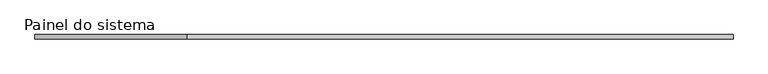
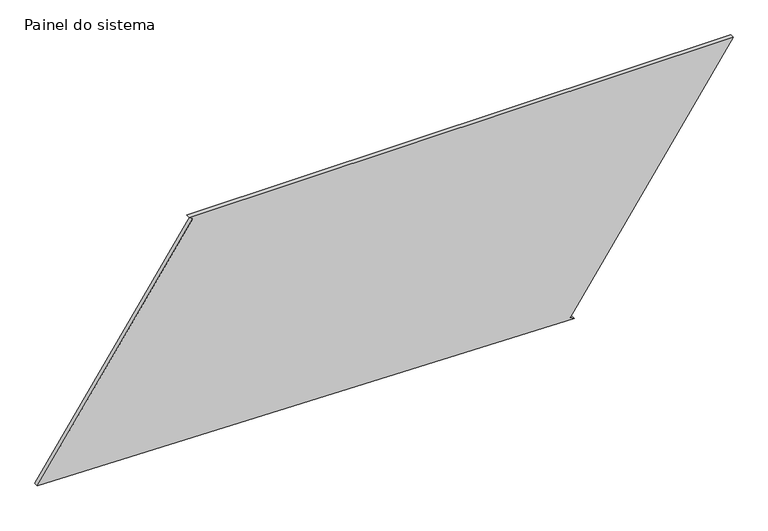
"""IFC4 building model written with IfcOpenShell, lengths in millimetres: plate geometry, Painel do sistema : Envidraçado."""

from ifc_helpers import new_model, si_unit, frame, origin, place, context, project, spatial, polyline, outline, extrude, source, transform, mapped, element, save


def painel_do_sistema_5d628f52(model_context):
    return source(origin(), model_context, "Body", "SweptSolid", [
        extrude(outline(polyline([(0.0, 1069.4494093), (14.052453, 1048.7726454), (1368.7753638, 1969.4766825), (1368.7753638, -1110.8275547), (1354.7229108, -1090.1507908), (60.8837577, -1969.4766825), (0.0, 1069.4494093)])), frame((0.0, 24.5, 0.0), z_axis=(0.0, 1.0, 0.0), x_axis=(0.0, 0.0, 1.0)), (0.0, 0.0, 1.0), 25.0),
    ])


if __name__ == "__main__":
    model = new_model("IFC4")
    model_context = context("Model", 3, world=origin())
    ifc_project = project(units=[si_unit("LENGTHUNIT", "METRE", prefix="MILLI")], contexts=[model_context])
    site = spatial("IfcSite", under=ifc_project)
    building = spatial("IfcBuilding", under=site)
    placement = place(None, origin())
    painel_do_sistema_shape = painel_do_sistema_5d628f52(model_context)
    element("IfcPlate", 1, ObjectType="Painel do sistema : Envidraçado", at=placement, inside=building, context=model_context, shape_type="MappedRepresentation", body=[
        mapped(painel_do_sistema_shape, transform((0.0, 0.0, 0.0), x_axis=(1.0, 0.0, 0.0), y_axis=(0.0, 1.0, 0.0), z_axis=(0.0, 0.0, 1.0))),
    ])
    save(model, "model.ifc")

# Revit data of these elements
# Type "Painel do sistema : Envidraçado"
#   Construction Type Id = "GSP4R"
#   Analytic Construction = "Vidraça única Pilkington 1/8 pol"
#   Visual Light Transmittance = 0.9
#   Solar Heat Gain Coefficient = 0.86
#   Heat Transfer Coefficient (U) = 6.7069 W/(m²·K)
# Element 1 (IfcPlate, "Painel do sistema : Envidraçado")
#   Materials on its faces: "Vidro"
# Materials
#   "Vidro": class "Vidro", colour RGB 0 128 192, transparency 0.9, Description = "Vidro de sílica", Cost = 0
